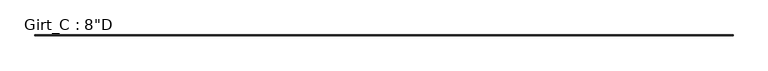
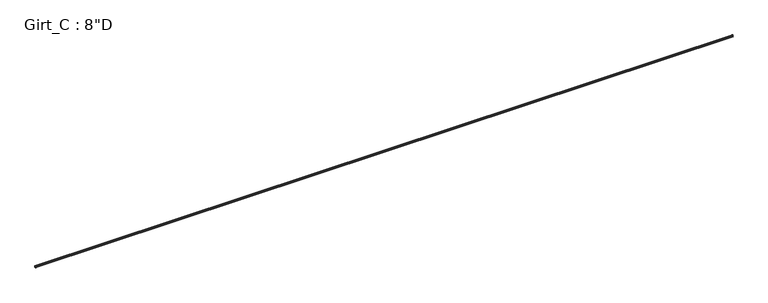
"""IFC4 building model written with IfcOpenShell, lengths in millimetres: beam geometry."""

from ifc_helpers import new_model, si_unit, point, frame, frame_2d, origin, place, context, project, spatial, polyline, circle_curve, trimmed, segment, composite_curve, outline, extrude, source, transform, mapped, element, save


def beam_34d67c3c(model_context):
    return source(origin(), model_context, "Body", "SweptSolid", [
        extrude(outline(composite_curve([segment(polyline([(-87.5109375, 101.6), (-3.3734375, 101.6)]), True, "CONTINUOUS"), segment(trimmed(circle_curve(frame_2d((-3.3734375, 96.8375)), 4.7625), [point((-3.3734375, 101.6))], [point((1.3890625, 96.8375))], False, "CARTESIAN"), True, "CONTINUOUS"), segment(polyline([(1.3890625, 96.8375), (1.3890625, -96.8375)]), True, "CONTINUOUS"), segment(trimmed(circle_curve(frame_2d((-3.3734375, -96.8375)), 4.7625), [point((1.3890625, -96.8375))], [point((-3.3734375, -101.6))], False, "CARTESIAN"), True, "CONTINUOUS"), segment(polyline([(-3.3734375, -101.6), (-87.5109375, -101.6), (-99.7792647, -86.979177), (-97.6510975, -85.1934327), (-86.2154765, -98.821875), (-3.2694106, -98.821875)]), True, "CONTINUOUS"), segment(trimmed(circle_curve(frame_2d((-3.3748024, -96.8389339)), 1.9857399), [point((-3.2694106, -98.821875))], [point((-1.3890625, -96.8389339))], True, "CARTESIAN"), True, "CONTINUOUS"), segment(polyline([(-1.3890625, -96.8389339), (-1.3890625, 96.8381931)]), True, "CONTINUOUS"), segment(trimmed(circle_curve(frame_2d((-3.3741066, 96.8381931)), 1.9850441), [point((-1.3890625, 96.8381931))], [point((-3.3005807, 98.821875))], True, "CARTESIAN"), True, "CONTINUOUS"), segment(polyline([(-3.3005807, 98.821875), (-86.2154765, 98.821875), (-97.6278742, 85.221109), (-99.7560415, 87.0068534), (-87.5109375, 101.6)]), True, "CONTINUOUS")], self_intersect=False)), frame((-44402.375, 0.0, 0.0), z_axis=(1.0, 0.0, 0.0), x_axis=(0.0, 1.0, 0.0)), (0.0, 0.0, 1.0), 88633.3),
    ])


if __name__ == "__main__":
    model = new_model("IFC4")
    model_context = context("Model", 3, world=origin())
    ifc_project = project(units=[si_unit("LENGTHUNIT", "METRE", prefix="MILLI")], contexts=[model_context])
    site = spatial("IfcSite", under=ifc_project)
    building = spatial("IfcBuilding", under=site)
    placement = place(None, origin())
    beam_shape = beam_34d67c3c(model_context)
    element("IfcBeam", 1, ObjectType="Girt_C : 8\"D", at=placement, inside=building, context=model_context, shape_type="MappedRepresentation", body=[
        mapped(beam_shape, transform((0.0, 0.0, 0.0), x_axis=(1.0, 0.0, 0.0), y_axis=(0.0, 1.0, 0.0), z_axis=(0.0, 0.0, 1.0))),
    ])
    save(model, "model.ifc")

# Revit data of these elements
# Type "Girt_C : 8\"D"
#   half leg = 0' - 1 3/4"
#   Web_Thickness = 0' - 0 7/64"
#   Length [instance default] = 10' - 0"
#   Leg_1 = 0' - 3 1/2"
#   Height = 0' - 8"
#   Structural Material [instance default] = none
# Element 1 (IfcBeam, "Girt_C : 8\"D")
#   Structural Material = CEE' SECTION (8.0x3.5C - SEE STRUCT. DWGS)
#   Materials on its faces: "CEE' SECTION (8.0x3.5C - SEE STRUCT. DWGS)"
# Materials
#   "CEE' SECTION (8.0x3.5C - SEE STRUCT. DWGS)": class "Metal", colour RGB 137 146 153, transparency 0, Description = "Steel, mill finish", Cost = 0
